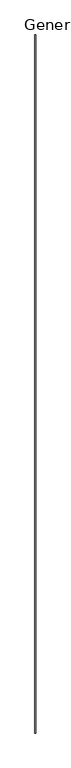
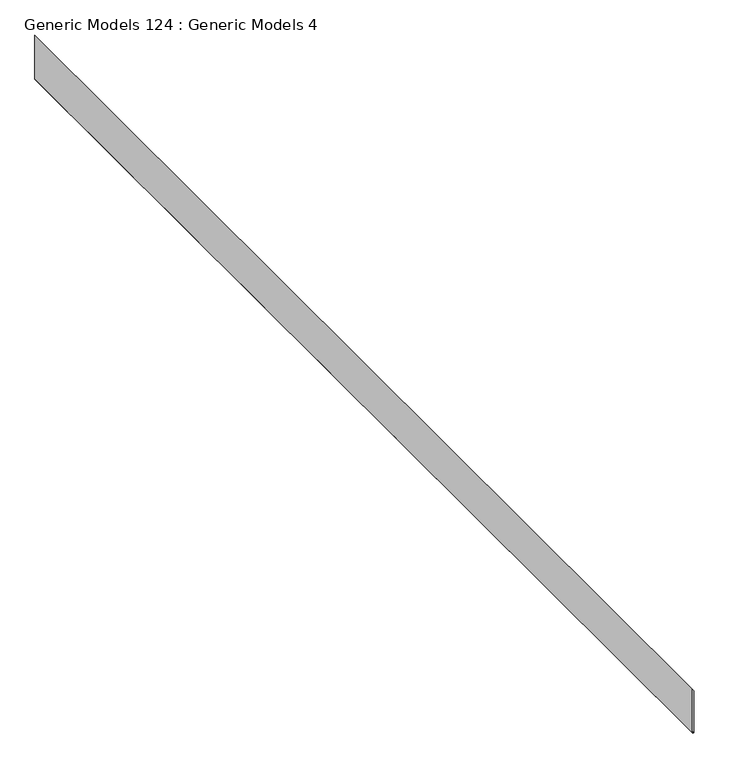
"""IFC4 building model written with IfcOpenShell, lengths in millimetres: proxy geometry, Generic Models 124 : Generic Models 4."""

from ifc_helpers import new_model, si_unit, frame, origin, place, context, project, spatial, polyline, outline, extrude, source, transform, mapped, element, save


def generic_models_124_generic_models_4_777518e4(model_context):
    return source(origin(), model_context, "Body", "SweptSolid", [
        extrude(outline(polyline([(126343.791, 7092.8674948), (127068.6707574, 7092.8674948), (127105.9455785, 7073.7263704), (126347.2708, 7073.7263704), (126347.2708, 7074.5852113), (126366.3153787, 7074.5852113), (126366.3153787, 7075.8552113), (126346.0008, 7075.8552113), (126346.0008, 7074.9963704), (126343.791, 7074.9963704), (126343.791, 7092.8674948)])), frame((0.0, -6864.9230338, 0.0), z_axis=(0.0, 1.0, 0.0), x_axis=(0.0, 0.0, 1.0)), (0.0, 0.0, 1.0), 18643.6),
    ])


if __name__ == "__main__":
    model = new_model("IFC4")
    model_context = context("Model", 3, world=origin())
    ifc_project = project(units=[si_unit("LENGTHUNIT", "METRE", prefix="MILLI")], contexts=[model_context])
    site = spatial("IfcSite", under=ifc_project)
    building = spatial("IfcBuilding", under=site)
    placement = place(None, origin())
    generic_models_124_generic_models_4_shape = generic_models_124_generic_models_4_777518e4(model_context)
    element("IfcBuildingElementProxy", 1, Name="Generic Models 124 : Generic Models 4", ObjectType="Generic Models 124 : Generic Models 4", at=placement, inside=building, context=model_context, shape_type="MappedRepresentation", body=[
        mapped(generic_models_124_generic_models_4_shape, transform((0.0, 0.0, 0.0), x_axis=(1.0, 0.0, 0.0), y_axis=(0.0, 1.0, 0.0), z_axis=(0.0, 0.0, 1.0))),
    ])
    save(model, "model.ifc")

# Revit data of these elements
# Element 1 (IfcBuildingElementProxy, "Generic Models 124 : Generic Models 4")
#   Materials on its faces: "_7/8\" SMOOTH TROWEL EXTERIOR STUCCO (COLOR PER OWNER)"
# Materials
#   "_7/8\" SMOOTH TROWEL EXTERIOR STUCCO (COLOR PER OWNER)": class "Generic", colour RGB 233 233 233, transparency 0, Cost = 0
